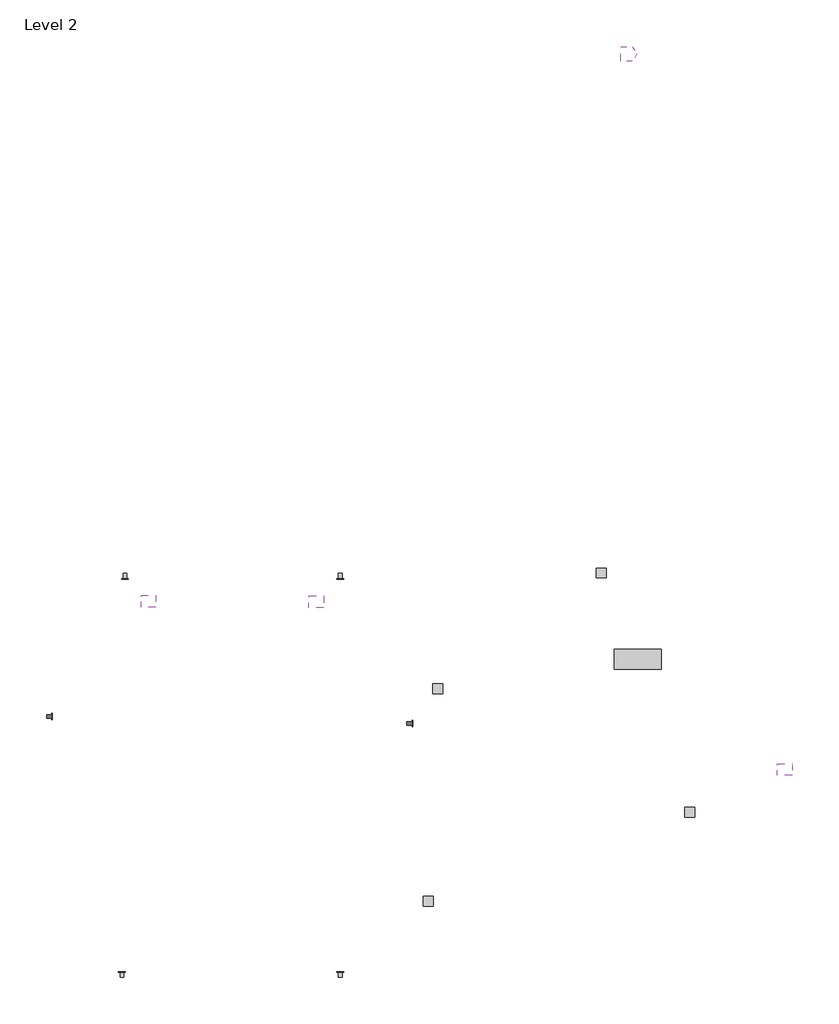
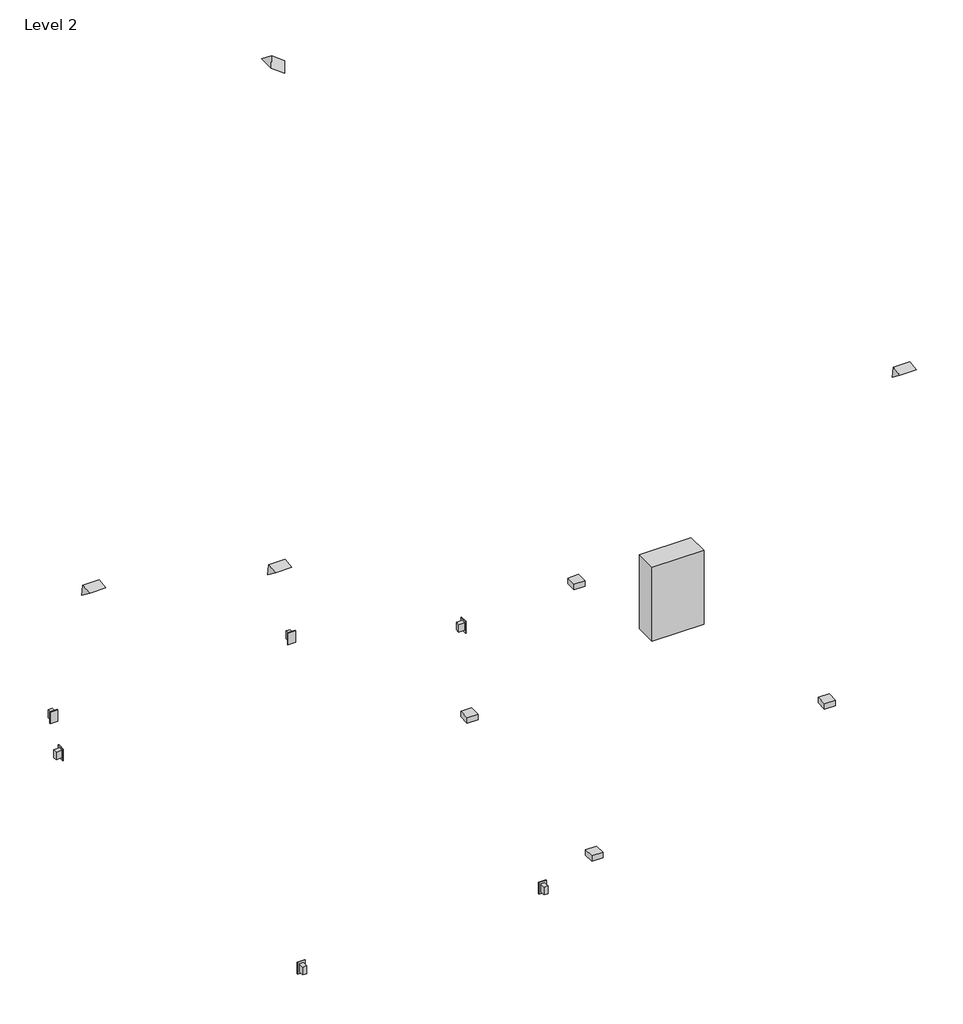
# One storey: 9 proxies, 4 light fixtures, 2 switching devices.
"""IFC4 building model written with IfcOpenShell, lengths in millimetres."""

import ifcopenshell
import ifcopenshell.guid

model = None  # the IFC model being written
_history = None  # IfcOwnerHistory: only IFC2X3 demands one
_inside = {}  # id of a spatial element -> (the spatial element, [elements in it])
_under = {}  # id of a project, library or spatial element -> (it, [spatial elements below it])
_declared = {}  # id of a project -> (the project, [libraries it declares])
_typed = {}  # id of a type object -> (the type object, [elements of that type])
_made_of = {}  # id of a material, layer set ... -> (it, [elements and type objects made of it])


def new_model(schema):
    """Start an empty IFC model of exactly this schema.

    Asked for "IFC4X3", IfcOpenShell would pick the latest addendum, in which some entities
    have other attributes; the version numbers below select the first issue.
    IFC2X3 requires an IfcOwnerHistory on every rooted entity: one is made here for all.
    """
    global model, _history
    if schema == "IFC4X3":
        model = ifcopenshell.file(schema_version=(4, 3, 0, 0))
    else:
        model = ifcopenshell.file(schema=schema)
    _inside.clear()
    _under.clear()
    _declared.clear()
    _typed.clear()
    _made_of.clear()
    _history = None
    if model.schema == "IFC2X3":
        org = make("IfcOrganization", Name="unknown")
        user = make(
            "IfcPersonAndOrganization",
            ThePerson=make("IfcPerson", FamilyName="unknown"),
            TheOrganization=org,
        )
        app = make(
            "IfcApplication",
            ApplicationDeveloper=org,
            Version="unknown",
            ApplicationFullName="unknown",
            ApplicationIdentifier="unknown",
        )
        _history = make(
            "IfcOwnerHistory",
            OwningUser=user,
            OwningApplication=app,
            ChangeAction="ADDED",
            CreationDate=0,
        )
    return model


def make(cls, **values):
    """One entity of the class cls with the attributes given. An attribute that is None is left unset."""
    return model.create_entity(
        cls, **{name: value for name, value in values.items() if value is not None}
    )


def rooted(cls, **values):
    """An entity with a GlobalId (a new one), such as an element, a storey or a relation."""
    return make(cls, GlobalId=ifcopenshell.guid.new(), OwnerHistory=_history, **values)


def si_unit(unit_type, name, prefix=None):
    """IfcSIUnit, for example si_unit("LENGTHUNIT", "METRE", prefix="MILLI")."""
    return make("IfcSIUnit", UnitType=unit_type, Prefix=prefix, Name=name)


def assignment(units):
    """IfcUnitAssignment: the units of a project."""
    return None if units is None else make("IfcUnitAssignment", Units=units)


def point(xyz):
    """IfcCartesianPoint."""
    return None if xyz is None else make("IfcCartesianPoint", Coordinates=xyz)


def direction(xyz):
    """IfcDirection."""
    return None if xyz is None else make("IfcDirection", DirectionRatios=xyz)


def frame(location, z_axis=None, x_axis=None):
    """IfcAxis2Placement3D, a coordinate frame: its origin and axes. An axis left out is left unset."""
    return make(
        "IfcAxis2Placement3D",
        Location=point(location),
        Axis=direction(z_axis),
        RefDirection=direction(x_axis),
    )


def origin():
    """The frame at (0, 0, 0) with its axes left unset."""
    return frame((0.0, 0.0, 0.0))


def origin_with_axes():
    """The frame at (0, 0, 0) with the z axis (0, 0, 1) and the x axis (1, 0, 0) written out."""
    return frame((0.0, 0.0, 0.0), z_axis=(0.0, 0.0, 1.0), x_axis=(1.0, 0.0, 0.0))


def place(relative_to, where):
    """IfcLocalPlacement: puts the frame where relative to a parent placement (None: the world)."""
    return make(
        "IfcLocalPlacement", PlacementRelTo=relative_to, RelativePlacement=where
    )


def context(
    kind, dimensions, precision=None, world=None, true_north=None, identifier=None
):
    """IfcGeometricRepresentationContext, for example the 3D "Model" context."""
    return make(
        "IfcGeometricRepresentationContext",
        ContextIdentifier=identifier,
        ContextType=kind,
        CoordinateSpaceDimension=dimensions,
        Precision=precision,
        WorldCoordinateSystem=world,
        TrueNorth=true_north,
    )


def project(units=None, contexts=None):
    """IfcProject with its units and contexts."""
    return rooted(
        "IfcProject",
        Name="project",
        RepresentationContexts=contexts,
        UnitsInContext=assignment(units),
    )


def spatial(cls, under=None, at=None, **own):
    """A site, building, storey or space (cls), placed at a placement, below another one or the project."""
    s = rooted(cls, ObjectPlacement=at, **own)
    if under is not None:
        _under.setdefault(under.id(), (under, []))[1].append(s)
    return s


def polyline(points):
    """IfcPolyline through the points."""
    return make("IfcPolyline", Points=[point(p) for p in points])


def outline(outer, holes=None, kind="AREA"):
    """IfcArbitraryClosedProfileDef: a profile drawn as a closed curve; with holes, ...WithVoids."""
    if holes is None:
        return make("IfcArbitraryClosedProfileDef", ProfileType=kind, OuterCurve=outer)
    return make(
        "IfcArbitraryProfileDefWithVoids",
        ProfileType=kind,
        OuterCurve=outer,
        InnerCurves=holes,
    )


def extrude(swept, where, along, depth):
    """IfcExtrudedAreaSolid: the profile swept, set in the frame where, extruded along a direction by depth."""
    return make(
        "IfcExtrudedAreaSolid",
        SweptArea=swept,
        Position=where,
        ExtrudedDirection=direction(along),
        Depth=depth,
    )


def shape(context_of_items, identifier, shape_type, items):
    """IfcShapeRepresentation: the items that make up one representation, for example the "Body"."""
    return make(
        "IfcShapeRepresentation",
        ContextOfItems=context_of_items,
        RepresentationIdentifier=identifier,
        RepresentationType=shape_type,
        Items=items,
    )


def source(mapping_origin, context_of_items, identifier, shape_type, items):
    """IfcRepresentationMap: a shape defined once, which mapped items show again and again."""
    return make(
        "IfcRepresentationMap",
        MappingOrigin=mapping_origin,
        MappedRepresentation=shape(context_of_items, identifier, shape_type, items),
    )


def transform(
    local_origin,
    x_axis=None,
    y_axis=None,
    z_axis=None,
    scale=None,
    scale2=None,
    scale3=None,
    uniform=True,
):
    """IfcCartesianTransformationOperator3D, or its non-uniform kind. x_axis, y_axis, z_axis: its Axis1, 2, 3."""
    if uniform:
        return make(
            "IfcCartesianTransformationOperator3D",
            Axis1=direction(x_axis),
            Axis2=direction(y_axis),
            LocalOrigin=point(local_origin),
            Scale=scale,
            Axis3=direction(z_axis),
        )
    return make(
        "IfcCartesianTransformationOperator3DnonUniform",
        Axis1=direction(x_axis),
        Axis2=direction(y_axis),
        LocalOrigin=point(local_origin),
        Scale=scale,
        Axis3=direction(z_axis),
        Scale2=scale2,
        Scale3=scale3,
    )


def mapped(mapping_source, mapping_target):
    """IfcMappedItem: shows the shape of a source again, moved by a transform."""
    return make(
        "IfcMappedItem", MappingSource=mapping_source, MappingTarget=mapping_target
    )


def made_of(thing, what):
    """Note that an element or type object is made of a material, layer set ...; save() writes the relation."""
    if what is not None:
        _made_of.setdefault(what.id(), (what, []))[1].append(thing)
    return thing


def element(
    cls,
    number,
    at=None,
    inside=None,
    cuts=None,
    type_object=None,
    material=None,
    context=None,
    identifier="Body",
    shape_type=None,
    held_by="IfcProductDefinitionShape",
    body=None,
    shapes=None,
    **own,
):
    """One element of the class cls, such as IfcWall. Its Tag is "e" and its number.

    at: its placement. inside: the storey or other place that contains it. cuts: it is an
    opening in that element (IfcRelVoidsElement). A single representation is given by context,
    identifier, shape_type and body (its items); several are given by shapes. held_by: the class
    of the entity that holds the representations. save() writes the other relations.
    """
    e = rooted(cls, Tag="e%d" % number, ObjectPlacement=at, **own)
    if body is not None:
        shapes = [shape(context, identifier, shape_type, body)]
    if shapes is not None:
        e.Representation = make(held_by, Representations=shapes)
    if inside is not None:
        _inside.setdefault(inside.id(), (inside, []))[1].append(e)
    if cuts is not None:
        rooted(
            "IfcRelVoidsElement", RelatingBuildingElement=cuts, RelatedOpeningElement=e
        )
    if type_object is not None:
        _typed.setdefault(type_object.id(), (type_object, []))[1].append(e)
    return made_of(e, material)


def aggregate(whole, parts):
    """IfcRelAggregates: a whole, such as a stair, and the parts it consists of."""
    return rooted("IfcRelAggregates", RelatingObject=whole, RelatedObjects=parts)


def save(model, path):
    """Write the relations noted so far, then the file.

    IfcRelAggregates (storeys below a building ...), IfcRelContainedInSpatialStructure (elements
    in a storey), IfcRelDefinesByType, IfcRelAssociatesMaterial and IfcRelDeclares: one each for
    every whole, place, type object, material and project.
    """
    for whole, parts in _under.values():
        aggregate(whole, parts)
    for where, things in _inside.values():
        rooted(
            "IfcRelContainedInSpatialStructure",
            RelatedElements=things,
            RelatingStructure=where,
        )
    for kind, things in _typed.values():
        rooted("IfcRelDefinesByType", RelatedObjects=things, RelatingType=kind)
    for what, things in _made_of.values():
        rooted("IfcRelAssociatesMaterial", RelatedObjects=things, RelatingMaterial=what)
    for by, libraries in _declared.values():
        rooted("IfcRelDeclares", RelatingContext=by, RelatedDefinitions=libraries)
    model.write(path)


def duplex_receptacle_gfci_10251bba(model_context):
    return source(origin(), model_context, "Body", "SweptSolid", [
        extrude(outline(polyline([(19.05, 38.1), (19.05, -38.1), (-19.05, -38.1), (-19.05, 38.1), (19.05, 38.1)])), frame((0.0, 0.0, -53.975), z_axis=(0.0, 0.0, 1.0), x_axis=(1.0, 0.0, 0.0)), (0.0, 0.0, 1.0), 53.975),
        extrude(outline(polyline([(34.925, 57.15), (34.925, -57.15), (-34.925, -57.15), (-34.925, 57.15), (34.925, 57.15)])), origin_with_axes(), (0.0, 0.0, 1.0), 4.7625),
    ])


def heater_standard_9b13520e(model_context):
    return source(origin(), model_context, "Body", "SweptSolid", [
        extrude(outline(polyline([(240.0101563, 0.0), (240.0101563, -203.2), (-240.0101562, -203.2), (-240.0101562, 0.0), (240.0101563, 0.0)])), origin_with_axes(), (0.0, 0.0, 1.0), 726.4796875),
    ])


def proxy_222d7609(model_context):
    return source(origin(), model_context, "Body", "SweptSolid", [
        extrude(outline(polyline([(50.8, 50.8), (50.8, -50.8), (-50.8, -50.8), (-50.8, 50.8), (50.8, 50.8)])), origin_with_axes(), (0.0, 0.0, 1.0), 53.975),
    ])


def plain_recessed_lighting_fixture_small_bulb_b229a362(model_context):
    return source(origin(), model_context, "Body", "SweptSolid", [
        extrude(outline(polyline([(-152.4, 0.0), (0.0, 0.0), (-76.2, -76.2), (-152.4, 0.0)])), frame((0.0, 0.0, 0.0), z_axis=(1.0, 0.0, 0.0), x_axis=(0.0, 1.0, 0.0)), (0.0, 0.0, 1.0), 152.4),
    ])


model = new_model("IFC4")

# Units and contexts
model_context = context("Model", 3, world=origin())
ifc_project = project(units=[si_unit("LENGTHUNIT", "METRE", prefix="MILLI")], contexts=[model_context])

# Site, building, storey
site = spatial("IfcSite", under=ifc_project)
building = spatial("IfcBuilding", under=site)
storey = spatial("IfcBuildingStorey", under=building, Name="Level 2", Elevation=3048.0)

# Proxies
placement = place(None, origin())
duplex_receptacle_gfci_shape = duplex_receptacle_gfci_10251bba(model_context)
element("IfcBuildingElementProxy", 1, Name="Duplex Receptacle : Standard", ObjectType="Duplex Receptacle : Standard", at=placement, inside=storey, context=model_context, shape_type="MappedRepresentation", body=[
    mapped(duplex_receptacle_gfci_shape, transform((-4722.187287, 5277.9871474, 3505.2), x_axis=(1.0, 0.0, 0.0), y_axis=(0.0, 0.0, 1.0), z_axis=(0.0, -1.0, 0.0))),
])
element("IfcBuildingElementProxy", 2, Name="Duplex Receptacle : Standard", ObjectType="Duplex Receptacle : Standard", at=placement, inside=storey, context=model_context, shape_type="MappedRepresentation", body=[
    mapped(duplex_receptacle_gfci_shape, transform((-2512.7582686, 5277.9871474, 3505.2), x_axis=(1.0, 0.0, 0.0), y_axis=(0.0, 0.0, 1.0), z_axis=(0.0, -1.0, 0.0))),
])
element("IfcBuildingElementProxy", 3, Name="Duplex Receptacle : Standard", ObjectType="Duplex Receptacle : Standard", at=placement, inside=storey, context=model_context, shape_type="MappedRepresentation", body=[
    mapped(duplex_receptacle_gfci_shape, transform((-2512.7582686, 1239.3871474, 3505.2), x_axis=(-1.0, 0.0, 0.0), y_axis=(0.0, 0.0, 1.0), z_axis=(0.0, 1.0, 0.0))),
])
element("IfcBuildingElementProxy", 4, Name="Duplex Receptacle : Standard", ObjectType="Duplex Receptacle : Standard", at=placement, inside=storey, context=model_context, shape_type="MappedRepresentation", body=[
    mapped(duplex_receptacle_gfci_shape, transform((-4754.4273183, 1239.3871474, 3505.2), x_axis=(-1.0, 0.0, 0.0), y_axis=(0.0, 0.0, 1.0), z_axis=(0.0, 1.0, 0.0))),
])
heater_standard_shape = heater_standard_9b13520e(model_context)
element("IfcBuildingElementProxy", 5, Name="Heater : Standard", ObjectType="Heater : Standard", at=placement, inside=storey, context=model_context, shape_type="MappedRepresentation", body=[
    mapped(heater_standard_shape, transform((538.599819, 4552.0319544, 3048.0), x_axis=(1.0, 0.0, 0.0), y_axis=(0.0, 1.0, 0.0), z_axis=(0.0, 0.0, 1.0))),
])
proxy_shape = proxy_222d7609(model_context)
element("IfcBuildingElementProxy", 6, Name="Junction Boxes - Load : 4\" Square 120 - 1", ObjectType="Junction Boxes - Load : 4\" Square 120 - 1", at=placement, inside=storey, context=model_context, shape_type="MappedRepresentation", body=[
    mapped(proxy_shape, transform((-1612.246226, 1968.9017872, 3048.0), x_axis=(1.0, 0.0, 0.0), y_axis=(0.0, 1.0, 0.0), z_axis=(0.0, 0.0, 1.0))),
])
element("IfcBuildingElementProxy", 7, Name="Junction Boxes - Load : 4\" Square 120 - 1", ObjectType="Junction Boxes - Load : 4\" Square 120 - 1", at=placement, inside=storey, context=model_context, shape_type="MappedRepresentation", body=[
    mapped(proxy_shape, transform((1074.7050896, 2881.2949551, 3048.0), x_axis=(1.0, 0.0, 0.0), y_axis=(0.0, 1.0, 0.0), z_axis=(0.0, 0.0, 1.0))),
])
element("IfcBuildingElementProxy", 8, Name="Junction Boxes - Load : 4\" Square 120 - 1", ObjectType="Junction Boxes - Load : 4\" Square 120 - 1", at=placement, inside=storey, context=model_context, shape_type="MappedRepresentation", body=[
    mapped(proxy_shape, transform((-1512.9191351, 4148.4516228, 3048.0), x_axis=(1.0, 0.0, 0.0), y_axis=(0.0, 1.0, 0.0), z_axis=(0.0, 0.0, 1.0))),
])
element("IfcBuildingElementProxy", 9, Name="Junction Boxes - Load : 4\" Square 120 - 1", ObjectType="Junction Boxes - Load : 4\" Square 120 - 1", at=placement, inside=storey, context=model_context, shape_type="MappedRepresentation", body=[
    mapped(proxy_shape, transform((166.2893189, 5336.4630461, 3048.0), x_axis=(1.0, 0.0, 0.0), y_axis=(0.0, 1.0, 0.0), z_axis=(0.0, 0.0, 1.0))),
])

# Light fixtures
plain_recessed_lighting_fixture_small_bulb_shape = plain_recessed_lighting_fixture_small_bulb_b229a362(model_context)
element("IfcLightFixture", 10, ObjectType="Plain Recessed Lighting Fixture : Small Bulb", at=placement, inside=storey, context=model_context, shape_type="MappedRepresentation", body=[
    mapped(plain_recessed_lighting_fixture_small_bulb_shape, transform((-4558.0249556, 4985.2608347, 4832.1739718), x_axis=(1.0, 0.0, 0.0), y_axis=(0.0, -0.8000000000000005, 0.5999999999999995), z_axis=(0.0, -0.5999999999999995, -0.8000000000000005))),
])
element("IfcLightFixture", 11, ObjectType="Plain Recessed Lighting Fixture : Small Bulb", at=placement, inside=storey, context=model_context, shape_type="MappedRepresentation", body=[
    mapped(plain_recessed_lighting_fixture_small_bulb_shape, transform((-2835.7010642, 4978.8236548, 4434.3345234), x_axis=(1.0, 0.0, 0.0), y_axis=(0.0, -0.8000000000000005, 0.5999999999999995), z_axis=(0.0, -0.5999999999999995, -0.8000000000000005))),
])
element("IfcLightFixture", 12, ObjectType="Plain Recessed Lighting Fixture : Small Bulb", at=placement, inside=storey, context=model_context, shape_type="MappedRepresentation", body=[
    mapped(plain_recessed_lighting_fixture_small_bulb_shape, transform((1972.1869623, 3258.6871474, 5733.1507494), x_axis=(1.0, 0.0, 0.0), y_axis=(0.0, -0.8000000000000005, 0.5999999999999995), z_axis=(0.0, -0.5999999999999995, -0.8000000000000005))),
])
element("IfcLightFixture", 13, ObjectType="Plain Recessed Lighting Fixture : Small Bulb", at=placement, inside=storey, context=model_context, shape_type="MappedRepresentation", body=[
    mapped(plain_recessed_lighting_fixture_small_bulb_shape, transform((363.8318219, 10586.8927854, 4866.0489868), x_axis=(0.8000000000000004, 0.0, -0.5999999999999995), y_axis=(0.0, -1.0, 0.0), z_axis=(-0.5999999999999995, 0.0, -0.8000000000000004))),
])

# Switching devices
element("IfcSwitchingDevice", 14, ObjectType="Lighting Switches : Single Pole", at=placement, inside=storey, context=model_context, shape_type="MappedRepresentation", body=[
    mapped(duplex_receptacle_gfci_shape, transform((-5473.789748, 3863.5651529, 4267.2), x_axis=(0.0, 1.0, 0.0), y_axis=(0.0, 0.0, 1.0), z_axis=(1.0, 0.0, 0.0))),
])
element("IfcSwitchingDevice", 15, ObjectType="Lighting Switches : Single Pole", at=placement, inside=storey, context=model_context, shape_type="MappedRepresentation", body=[
    mapped(duplex_receptacle_gfci_shape, transform((-1774.914748, 3792.4947606, 4267.2), x_axis=(0.0, 1.0, 0.0), y_axis=(0.0, 0.0, 1.0), z_axis=(1.0, 0.0, 0.0))),
])

save(model, "model.ifc")

# Revit data of these elements
# Type "Duplex Receptacle : Standard"
#   Label = ""
#   Switch Voltage = 120 V
#   Load = 180 VA
#   Default Elevation = 1' - 6"
#   Load Classification = Receptacle
#   Assembly Code = ""
# Type "Heater : Standard"
#   Label = "H"
#   Width = 0' - 8"
#   Voltage = 120 V
#   Length = 1' - 6 115/128"
#   Height = 2' - 4 77/128"
#   Apparent Load = 1500 VA
#   Number of Poles = 1
#   Load Classification = Heating
#   Heater Material = none
#   Default Elevation = 0
# Type "Junction Boxes - Load : 4\" Square 120 - 1"
#   Width = 0' - 4"
#   Voltage = 120 V
#   Power Factor [instance default] = 1
#   Load [instance default] = 500 VA
#   Height = 0' - 4"
#   Depth = 0' - 2 1/8"
#   Number of Poles = 1
#   Load Classification = Power
#   Default Elevation = 0
# Type "Plain Recessed Lighting Fixture : Small Bulb"
#   Photometric Web File = "2x22UA12.ies"
#   Width = 0' - 6"
#   Wattage = 62 W
#   built-in parameter 1150110 = 1 (stored number, unit not read)
#   built-in parameter 1150109 = 1 (stored number, unit not read)
#   built-in parameter 1150113 = 1 (stored number, unit not read)
#   Tilt Angle = -90.00°
#   Lumens = 5199.94 lm
#   built-in parameter 1114217 = 0.88 (stored number, unit not read)
#   built-in parameter 1150115 = 1 (stored number, unit not read)
#   built-in parameter 1150105 = 413.798 (stored number, unit not read)
#   Length = 0' - 6"
#   built-in parameter 1150112 = 1 (stored number, unit not read)
#   built-in parameter 1150114 = 1 (stored number, unit not read)
#   built-in parameter 1150107 = 4230 (stored number, unit not read)
#   built-in parameter 1150106 = 4.13798 (stored number, unit not read)
#   Emit from Rectangle Width = 0' - 6"
#   Emit from Rectangle Length = 0' - 6"
#   built-in parameter 1150104 = 7.79178 (stored number, unit not read)
#   Depth = 0' - 6"
#   Default Elevation = 4' - 0"
#   Ballast Voltage = 120 V
#   built-in parameter 1114218 = 0.88 (stored number, unit not read)
#   built-in parameter 1150133 = 10 (stored number, unit not read)
#   Apparent Load = 62 VA
#   built-in parameter 1150134 = 8
#   built-in parameter 1150137 = 1
#   Color Filter = 16777215
#   built-in parameter 1140040 [instance default] = 1
#   Load Classification = Lighting - Dwelling Unit
#   Emit Shape Visible in Rendering = no
#   Dimming Lamp Color Temperature Shift = (empty or 0)
#   Assembly Code = ""
# Type "Lighting Switches : Single Pole"
#   Label = ""
#   Switch Voltage [instance default] = 120 V
#   Default Elevation = 4' - 0"
#   Apparent Load = 0 VA
#   Load Classification = Other
#   Assembly Code = ""
# Element 1 (IfcBuildingElementProxy, "Duplex Receptacle : Standard")
#   Mark = "36"
#   Phase Created = New Construction
# Element 2 (IfcBuildingElementProxy, "Duplex Receptacle : Standard")
#   Mark = "37"
#   Phase Created = New Construction
# Element 3 (IfcBuildingElementProxy, "Duplex Receptacle : Standard")
#   Mark = "38"
#   Phase Created = New Construction
# Element 4 (IfcBuildingElementProxy, "Duplex Receptacle : Standard")
#   Mark = "39"
#   Phase Created = New Construction
# Element 5 (IfcBuildingElementProxy, "Heater : Standard")
#   Mark = "42"
#   Phase Created = New Construction
# Element 6 (IfcBuildingElementProxy, "Junction Boxes - Load : 4\" Square 120 - 1")
#   Mark = "27"
#   Power Factor = 1
#   Load = 500 VA
#   Phase Created = New Construction
# Element 7 (IfcBuildingElementProxy, "Junction Boxes - Load : 4\" Square 120 - 1")
#   Mark = "28"
#   Power Factor = 1
#   Load = 500 VA
#   Phase Created = New Construction
# Element 8 (IfcBuildingElementProxy, "Junction Boxes - Load : 4\" Square 120 - 1")
#   Mark = "40"
#   Power Factor = 1
#   Load = 500 VA
#   Phase Created = New Construction
# Element 9 (IfcBuildingElementProxy, "Junction Boxes - Load : 4\" Square 120 - 1")
#   Mark = "41"
#   Power Factor = 1
#   Load = 500 VA
#   Phase Created = New Construction
# Element 10 (IfcLightFixture, "Plain Recessed Lighting Fixture : Small Bulb")
#   Mark = "5"
#   built-in parameter 1140040 = 1
#   Phase Created = New Construction
# Element 11 (IfcLightFixture, "Plain Recessed Lighting Fixture : Small Bulb")
#   Mark = "6"
#   built-in parameter 1140040 = 1
#   Phase Created = New Construction
# Element 12 (IfcLightFixture, "Plain Recessed Lighting Fixture : Small Bulb")
#   Mark = "7"
#   built-in parameter 1140040 = 1
#   Phase Created = New Construction
# Element 13 (IfcLightFixture, "Plain Recessed Lighting Fixture : Small Bulb")
#   Mark = "8"
#   built-in parameter 1140040 = 1
#   Phase Created = New Construction
# Element 14 (IfcSwitchingDevice, "Lighting Switches : Single Pole")
#   Mark = "12"
#   Switch Voltage = 120 V
#   Phase Created = New Construction
# Element 15 (IfcSwitchingDevice, "Lighting Switches : Single Pole")
#   Mark = "13"
#   Switch Voltage = 120 V
#   Phase Created = New Construction
